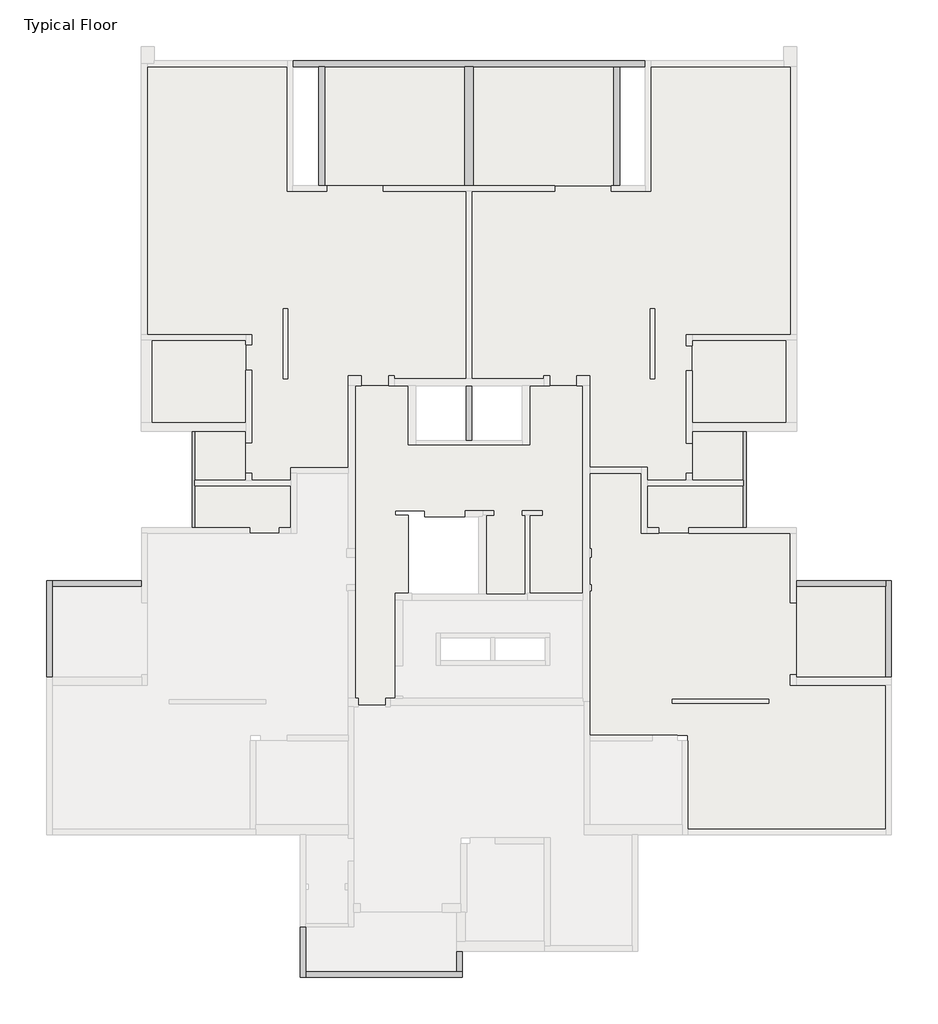
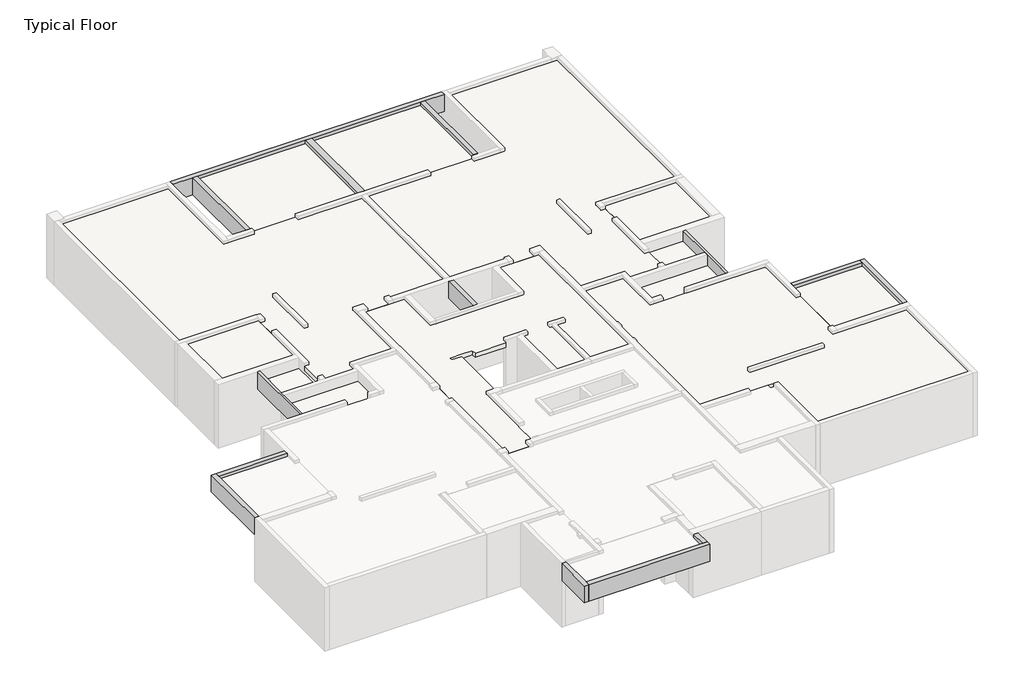
# One storey, part 4 of 4: 14 beams, 13 slabs.
"""IFC4 building model written with IfcOpenShell, lengths in millimetres."""

from ifc_helpers import new_model, si_unit, frame, origin, place, context, project, spatial, polyline, outline, extrude, faceted_brep, element, save

model = new_model("IFC4")

# Units and contexts
model_context = context("Model", 3, world=origin())
ifc_project = project(units=[si_unit("LENGTHUNIT", "METRE", prefix="MILLI")], contexts=[model_context])

# Site, building, storey
site = spatial("IfcSite", under=ifc_project)
building = spatial("IfcBuilding", under=site)
storey = spatial("IfcBuildingStorey", under=building, Name="Typical Floor", Elevation=3160.0)

# Beams
placement = place(None, origin())
element("IfcBeam", 1, ObjectType="Concrete Rectengular Beam : 10/80", at=placement, inside=storey, context=model_context, shape_type="Brep", body=[
    faceted_brep([(-4927.8090865, 3048.3506111, 3160.0), (-5027.8090865, 3048.3506111, 3160.0), (-5027.8090865, -271.5347538, 3160.0), (-4927.8090865, -271.5347538, 3160.0), (-4927.8090865, 1164.6693841, 3160.0), (-4927.8090865, 1364.6693841, 3160.0), (-4927.8090865, 3048.3506111, 2360.0), (-4927.8090865, 3048.3506111, 2510.0), (-4927.8090865, 3048.3506111, 2660.0), (-4927.8090865, -271.5347538, 2660.0), (-4927.8090865, -271.5347538, 2510.0), (-4927.8090865, -271.5347538, 2360.0), (-5027.8090865, 3048.3506111, 2360.0), (-5027.8090865, -271.5347538, 2360.0)], [[[0, 1, 2, 3, 4, 5]], [[6, 7, 8, 0, 5, 4, 3, 9, 10, 11]], [[12, 6, 11, 13]], [[1, 12, 13, 2]], [[1, 0, 8, 7, 6, 12]], [[3, 2, 13, 11, 10, 9]]]),
])
element("IfcBeam", 2, ObjectType="Concrete Rectengular Beam : 10/80", at=placement, inside=storey, context=model_context, shape_type="Brep", body=[
    faceted_brep([(14076.960118, 3048.3506111, 3160.0), (13976.960118, 3048.3506111, 3160.0), (13976.960118, 1364.6693841, 3160.0), (13976.960118, 1164.6693841, 3160.0), (13976.960118, -271.5348131, 3160.0), (14076.960118, -271.5348131, 3160.0), (14076.960118, 3048.3506111, 2360.0), (14076.960118, -271.5348131, 2360.0), (13976.960118, 3048.3506111, 2360.0), (13976.960118, -271.5348131, 2360.0), (13976.960118, 3048.3506111, 2660.0), (13976.960118, 3048.3506111, 2510.0), (13976.960118, -271.5348131, 2510.0), (13976.960118, -271.5348131, 2660.0)], [[[0, 1, 2, 3, 4, 5]], [[6, 0, 5, 7]], [[8, 6, 7, 9]], [[1, 10, 11, 8, 9, 12, 13, 4, 3, 2]], [[1, 0, 6, 8, 11, 10]], [[5, 4, 13, 12, 9, 7]]]),
])
element("IfcBeam", 3, ObjectType="Concrete Rectengular Beam : 20/80", at=placement, inside=storey, context=model_context, shape_type="Brep", body=[
    faceted_brep([(-9845.3223417, -2097.6508085, 3160.0), (-10045.3223417, -2097.6508085, 3160.0), (-10045.3223417, -5427.6243159, 3160.0), (-9845.3223417, -5427.6243159, 3160.0), (-9845.3223417, -2297.6508085, 3160.0), (-9845.3223417, -2097.6508085, 2360.0), (-9845.3223417, -5427.6243159, 3010.0), (-9845.3223417, -5427.6243159, 2810.0), (-9845.3223417, -5427.6243159, 2360.0), (-9845.3223417, -2297.6508085, 2360.0), (-10045.3223417, -2097.6508085, 2360.0), (-10045.3223417, -5427.6243159, 2360.0)], [[[0, 1, 2, 3, 4]], [[5, 0, 4, 3, 6, 7, 8, 9]], [[10, 5, 9, 8, 11]], [[1, 10, 11, 2]], [[1, 0, 5, 10]], [[3, 2, 11, 8, 7, 6]]]),
])
element("IfcBeam", 4, ObjectType="Concrete Rectengular Beam : 20/80", at=placement, inside=storey, context=model_context, shape_type="Brep", body=[
    faceted_brep([(-6765.3223417, -2097.6508085, 3160.0), (-6765.3223417, -2297.6508085, 3160.0), (-6765.3223417, -2297.6508085, 2360.0), (-6765.3223417, -2097.6508085, 2360.0), (-9845.3223417, -2097.6508085, 3160.0), (-9845.3223417, -2297.6508085, 3160.0), (-9845.3223417, -2297.6508085, 3010.0), (-9845.3223417, -2297.6508085, 2810.0), (-9845.3223417, -2297.6508085, 2360.0), (-9845.3223417, -2097.6508085, 2360.0)], [[[0, 1, 2, 3]], [[1, 0, 4, 5]], [[2, 1, 5, 6, 7, 8]], [[3, 2, 8, 9]], [[0, 3, 9, 4]], [[5, 4, 9, 8, 7, 6]]]),
])
element("IfcBeam", 5, ObjectType="Concrete Rectengular Beam : 20/80", at=placement, inside=storey, context=model_context, shape_type="Brep", body=[
    faceted_brep([(19089.4302812, -2097.6508085, 3160.0), (18889.4302812, -2097.6508085, 3160.0), (18889.4302812, -2297.6508085, 3160.0), (18889.4302812, -5431.5348131, 3160.0), (19089.4302812, -5431.5348131, 3160.0), (19089.4302812, -2097.6508085, 2360.0), (19089.4302812, -5431.5348131, 2360.0), (18889.4302812, -2097.6508085, 2360.0), (18889.4302812, -5431.5348131, 2360.0), (18889.4302812, -2297.6508085, 2360.0), (18889.4302812, -5431.5348131, 2810.0), (18889.4302812, -5431.5348131, 3010.0)], [[[0, 1, 2, 3, 4]], [[5, 0, 4, 6]], [[7, 5, 6, 8, 9]], [[1, 7, 9, 8, 10, 11, 3, 2]], [[1, 0, 5, 7]], [[4, 3, 11, 10, 8, 6]]]),
])
element("IfcBeam", 6, ObjectType="Concrete Rectengular Beam : 20/80", at=placement, inside=storey, context=model_context, shape_type="Brep", body=[
    faceted_brep([(15808.1220541, -2097.6508085, 3160.0), (15808.1220541, -2297.6508085, 3160.0), (18889.4302812, -2297.6508085, 3160.0), (18889.4302812, -2097.6508085, 3160.0), (15808.1220541, -2097.6508085, 2360.0), (18889.4302812, -2097.6508085, 2360.0), (15808.1220541, -2297.6508085, 2360.0), (18889.4302812, -2297.6508085, 2360.0), (15808.1220541, -2297.6508085, 3010.0), (15808.1220541, -2297.6508085, 2810.0), (18889.4302812, -2297.6508085, 2810.0), (18889.4302812, -2297.6508085, 3010.0)], [[[0, 1, 2, 3]], [[4, 0, 3, 5]], [[6, 4, 5, 7]], [[1, 8, 9, 6, 7, 10, 11, 2]], [[1, 0, 4, 6, 9, 8]], [[3, 2, 11, 10, 7, 5]]]),
])
element("IfcBeam", 7, ObjectType="Concrete Rectengular Beam : 20/80", at=placement, inside=storey, context=model_context, shape_type="Brep", body=[
    faceted_brep([(-1304.0660316, -15783.8829405, 3160.0), (-1104.0660316, -15783.8829405, 3160.0), (-1104.0660316, -15583.8829405, 3160.0), (-1104.0660316, -14027.6329213, 3160.0), (-1304.0660316, -14027.6329213, 3160.0), (-1304.0660316, -15783.8829405, 2360.0), (-1304.0660316, -14027.6329213, 2360.0), (-1104.0660316, -15783.8829405, 2360.0), (-1104.0660316, -14027.6329213, 2360.0), (-1104.0660316, -15583.8829405, 2360.0), (-1104.0660316, -14027.6329213, 2810.0), (-1104.0660316, -14027.6329213, 3010.0)], [[[0, 1, 2, 3, 4]], [[5, 0, 4, 6]], [[7, 5, 6, 8, 9]], [[1, 7, 9, 8, 10, 11, 3, 2]], [[4, 3, 11, 10, 8, 6]], [[1, 0, 5, 7]]]),
])
element("IfcBeam", 8, ObjectType="Concrete Rectengular Beam : 20/80", at=placement, inside=storey, context=model_context, shape_type="Brep", body=[
    faceted_brep([(4293.8641143, -15783.8829405, 3160.0), (4293.8641143, -15583.8829405, 3160.0), (4093.8641143, -15583.8829405, 3160.0), (-1104.0660316, -15583.8829405, 3160.0), (-1104.0660316, -15783.8829405, 3160.0), (4293.8641143, -15783.8829405, 2360.0), (-1104.0660316, -15783.8829405, 2360.0), (4293.8641143, -15583.8829405, 2360.0), (-1104.0660316, -15583.8829405, 2360.0), (4093.8641143, -15583.8829405, 2360.0), (-1104.0660316, -15583.8829405, 2810.0), (-1104.0660316, -15583.8829405, 3010.0)], [[[0, 1, 2, 3, 4]], [[5, 0, 4, 6]], [[7, 5, 6, 8, 9]], [[1, 7, 9, 8, 10, 11, 3, 2]], [[1, 0, 5, 7]], [[4, 3, 11, 10, 8, 6]]]),
])
element("IfcBeam", 9, ObjectType="Concrete Rectengular Beam : 20/80", at=placement, inside=storey, context=model_context, shape_type="Brep", body=[
    faceted_brep([(4293.8641143, -14884.0137597, 3160.0), (4093.8641143, -14884.0137597, 3160.0), (4093.8641143, -15583.8829405, 3160.0), (4293.8641143, -15583.8829405, 3160.0), (4293.8641143, -14884.0137597, 2360.0), (4293.8641143, -15583.8829405, 2360.0), (4093.8641143, -14884.0137597, 2360.0), (4093.8641143, -15583.8829405, 2360.0), (4093.8641143, -15583.8829405, 2810.0), (4093.8641143, -15583.8829405, 3010.0)], [[[0, 1, 2, 3]], [[4, 0, 3, 5]], [[6, 4, 5, 7]], [[1, 6, 7, 8, 9, 2]], [[1, 0, 4, 6]], [[3, 2, 9, 8, 7, 5]]]),
])
element("IfcBeam", 10, ObjectType="Concrete Rectengular Beam : 20/80", at=placement, inside=storey, context=model_context, shape_type="Brep", body=[
    faceted_brep([(-1550.9499448, 15824.626844, 3160.0), (-1550.9499448, 15624.626844, 3160.0), (-650.9499448, 15624.626844, 3160.0), (-450.9499448, 15624.626844, 3160.0), (4369.0500552, 15624.626844, 3160.0), (4669.0500552, 15624.626844, 3160.0), (9515.057825, 15624.626844, 3160.0), (9715.057825, 15624.626844, 3160.0), (10595.057825, 15624.626844, 3160.0), (10595.057825, 15824.626844, 3160.0), (-1550.9499448, 15624.626844, 2360.0), (-650.9499448, 15624.626844, 2360.0), (-450.9499448, 15624.626844, 2360.0), (4369.0500552, 15624.626844, 2360.0), (4669.0500552, 15624.626844, 2360.0), (9515.057825, 15624.626844, 2360.0), (9715.057825, 15624.626844, 2360.0), (10595.057825, 15624.626844, 2360.0), (-1550.9499448, 15824.626844, 2360.0), (10595.057825, 15824.626844, 2360.0)], [[[0, 1, 2, 3, 4, 5, 6, 7, 8, 9]], [[1, 10, 11, 12, 13, 14, 15, 16, 17, 8, 7, 6, 5, 4, 3, 2]], [[10, 18, 19, 17, 16, 15, 14, 13, 12, 11]], [[18, 0, 9, 19]], [[1, 0, 18, 10]], [[9, 8, 17, 19]]]),
])
element("IfcBeam", 11, ObjectType="Concrete Rectengular Beam : 20/80", at=placement, inside=storey, context=model_context, shape_type="Brep", body=[
    faceted_brep([(-650.9499448, 11524.9195447, 3160.0), (-450.9499448, 11524.9195447, 3160.0), (-450.9499448, 15624.626844, 3160.0), (-650.9499448, 15624.626844, 3160.0), (-650.9499448, 11524.9195447, 2360.0), (-650.9499448, 15624.626844, 2360.0), (-450.9499448, 11524.9195447, 2360.0), (-450.9499448, 15624.626844, 2360.0), (-450.9499448, 11524.9195447, 3010.0), (-450.9499448, 11524.9195447, 2810.0), (-450.9499448, 15624.626844, 2810.0), (-450.9499448, 15624.626844, 3010.0)], [[[0, 1, 2, 3]], [[4, 0, 3, 5]], [[6, 4, 5, 7]], [[1, 8, 9, 6, 7, 10, 11, 2]], [[1, 0, 4, 6, 9, 8]], [[3, 2, 11, 10, 7, 5]]]),
])
element("IfcBeam", 12, ObjectType="Concrete Rectengular Beam : 20/80", at=placement, inside=storey, context=model_context, shape_type="Brep", body=[
    faceted_brep([(9515.057825, 11524.9195447, 3160.0), (9715.057825, 11524.9195447, 3160.0), (9715.057825, 15624.626844, 3160.0), (9515.057825, 15624.626844, 3160.0), (9515.057825, 11524.9195447, 2360.0), (9515.057825, 11524.9195447, 2810.0), (9515.057825, 11524.9195447, 3010.0), (9515.057825, 15624.626844, 3010.0), (9515.057825, 15624.626844, 2810.0), (9515.057825, 15624.626844, 2360.0), (9715.057825, 11524.9195447, 2360.0), (9715.057825, 15624.626844, 2360.0)], [[[0, 1, 2, 3]], [[4, 5, 6, 0, 3, 7, 8, 9]], [[10, 4, 9, 11]], [[1, 10, 11, 2]], [[1, 0, 6, 5, 4, 10]], [[3, 2, 11, 9, 8, 7]]]),
])
element("IfcBeam", 13, ObjectType="Concrete Rectengular Beam : 20/80", at=placement, inside=storey, context=model_context, shape_type="SweptSolid", body=[
    extrude(outline(polyline([(4422.0544149, 4615.5631538), (4622.0544149, 4615.5631538), (4622.0544149, 2732.4743311), (4422.0544149, 2732.4743311), (4422.0544149, 4615.5631538)])), frame((0.0, 0.0, 2360.0), z_axis=(0.0, 0.0, 1.0), x_axis=(1.0, 0.0, 0.0)), (0.0, 0.0, 1.0), 800.0),
])
element("IfcBeam", 14, ObjectType="Concrete Rectengular Beam : 30/80", at=placement, inside=storey, context=model_context, shape_type="Brep", body=[
    faceted_brep([(4369.0500552, 11524.9195447, 3160.0), (4669.0500552, 11524.9195447, 3160.0), (4669.0500552, 15624.626844, 3160.0), (4369.0500552, 15624.626844, 3160.0), (4369.0500552, 11524.9195447, 2360.0), (4369.0500552, 11524.9195447, 2810.0), (4369.0500552, 11524.9195447, 3010.0), (4369.0500552, 15624.626844, 3010.0), (4369.0500552, 15624.626844, 2810.0), (4369.0500552, 15624.626844, 2360.0), (4669.0500552, 11524.9195447, 2360.0), (4669.0500552, 15624.626844, 2360.0), (4669.0500552, 11524.9195447, 3010.0), (4669.0500552, 11524.9195447, 2810.0), (4669.0500552, 15624.626844, 2810.0), (4669.0500552, 15624.626844, 3010.0)], [[[0, 1, 2, 3]], [[4, 5, 6, 0, 3, 7, 8, 9]], [[10, 4, 9, 11]], [[1, 12, 13, 10, 11, 14, 15, 2]], [[1, 0, 6, 5, 4, 10, 13, 12]], [[3, 2, 15, 14, 11, 9, 8, 7]]]),
])

# Slabs
element("IfcSlab", 15, ObjectType="D=20", at=placement, inside=storey, context=model_context, shape_type="Brep", body=[
    faceted_brep([(18889.4302812, -10669.1739201, 2810.0), (12069.8374389, -10669.1739201, 2810.0), (12069.8374389, -7625.251138, 2810.0), (12069.8374389, -7425.251138, 2810.0), (11709.8374389, -7425.251138, 2810.0), (10849.2361919, -7425.251138, 2810.0), (8689.2361919, -7425.251138, 2810.0), (8689.2361919, -2440.6761415, 2810.0), (8740.4562765, -2440.6761415, 2810.0), (8740.4562765, -2240.6761415, 2810.0), (8689.2361919, -2240.6761415, 2810.0), (8689.2361919, -1298.8355577, 2810.0), (8740.4562765, -1298.8355577, 2810.0), (8740.4562765, -998.8355577, 2810.0), (8689.2361919, -998.8355577, 2810.0), (8689.2361919, 1602.6523966, 2810.0), (8692.9791875, 1602.6523966, 2810.0), (10462.1205752, 1602.6523966, 2810.0), (10462.1205752, -471.5348131, 2810.0), (10662.1205752, -471.5348131, 2810.0), (11062.1205752, -471.5348131, 2810.0), (12108.1220541, -471.5348131, 2810.0), (15608.1220541, -471.5348131, 2810.0), (15608.1220541, -2868.5711301, 2810.0), (15808.1220541, -2868.5711301, 2810.0), (15808.1220541, -5351.6580536, 2810.0), (15608.1220541, -5351.6580536, 2810.0), (15608.1220541, -5711.5348131, 2810.0), (15808.1220541, -5711.5348131, 2810.0), (18889.4302812, -5711.5348131, 2810.0), (11536.8984681, -6331.4817686, 2810.0), (14866.281411, -6331.4817686, 2810.0), (14866.281411, -6181.4817686, 2810.0), (11536.8984681, -6181.4817686, 2810.0), (12069.8374389, -10669.1739201, 3010.0), (18889.4302812, -10669.1739201, 3010.0), (18889.4302812, -5711.5348131, 3010.0), (15808.1220541, -5711.5348131, 3010.0), (15608.1220541, -5711.5348131, 3010.0), (15608.1220541, -5351.6580536, 3010.0), (15808.1220541, -5351.6580536, 3010.0), (15808.1220541, -2868.5711301, 3010.0), (15608.1220541, -2868.5711301, 3010.0), (15608.1220541, -471.5348131, 3010.0), (12108.1220541, -471.5348131, 3010.0), (11062.1205752, -471.5348131, 3010.0), (10662.1205752, -471.5348131, 3010.0), (10462.1205752, -471.5348131, 3010.0), (10462.1205752, 1602.6523966, 3010.0), (8692.9791875, 1602.6523966, 3010.0), (8689.2361919, 1602.6523966, 3010.0), (8689.2361919, -998.8355577, 3010.0), (8740.4562765, -998.8355577, 3010.0), (8740.4562765, -1298.8355577, 3010.0), (8689.2361919, -1298.8355577, 3010.0), (8689.2361919, -2240.6761415, 3010.0), (8740.4562765, -2240.6761415, 3010.0), (8740.4562765, -2440.6761415, 3010.0), (8689.2361919, -2440.6761415, 3010.0), (8689.2361919, -7425.251138, 3010.0), (10849.2361919, -7425.251138, 3010.0), (11709.8374389, -7425.251138, 3010.0), (12069.8374389, -7425.251138, 3010.0), (12069.8374389, -7625.251138, 3010.0), (14866.281411, -6331.4817686, 3010.0), (11536.8984681, -6331.4817686, 3010.0), (11536.8984681, -6181.4817686, 3010.0), (14866.281411, -6181.4817686, 3010.0)], [[[0, 1, 2, 3, 4, 5, 6, 7, 8, 9, 10, 11, 12, 13, 14, 15, 16, 17, 18, 19, 20, 21, 22, 23, 24, 25, 26, 27, 28, 29], [30, 31, 32, 33]], [[34, 35, 36, 37, 38, 39, 40, 41, 42, 43, 44, 45, 46, 47, 48, 49, 50, 51, 52, 53, 54, 55, 56, 57, 58, 59, 60, 61, 62, 63], [64, 65, 66, 67]], [[1, 0, 35, 34]], [[1, 34, 63, 62, 3, 2]], [[3, 62, 61, 60, 59, 6, 5, 4]], [[7, 6, 59, 58]], [[8, 7, 58, 57]], [[9, 8, 57, 56]], [[10, 9, 56, 55]], [[11, 10, 55, 54]], [[12, 11, 54, 53]], [[13, 12, 53, 52]], [[14, 13, 52, 51]], [[15, 14, 51, 50]], [[16, 15, 50, 49]], [[17, 16, 49, 48]], [[18, 17, 48, 47]], [[18, 47, 46, 45, 44, 43, 22, 21, 20, 19]], [[23, 22, 43, 42]], [[24, 23, 42, 41]], [[25, 24, 41, 40]], [[26, 25, 40, 39]], [[27, 26, 39, 38]], [[27, 38, 37, 36, 29, 28]], [[0, 29, 36, 35]], [[31, 30, 65, 64]], [[33, 32, 67, 66]], [[32, 31, 64, 67]], [[30, 33, 66, 65]]]),
])
element("IfcSlab", 16, ObjectType="D=20", at=placement, inside=storey, context=model_context, shape_type="Brep", body=[
    faceted_brep([(6609.8903055, 2582.4743311, 2810.0), (6609.8903055, 4615.5631538, 2810.0), (7104.8461452, 4615.5631538, 2810.0), (7304.8461452, 4615.5631538, 2810.0), (8239.2361919, 4615.5631538, 2810.0), (8239.2361919, 4613.0861241, 2810.0), (8439.2361919, 4613.0861241, 2810.0), (8439.2361919, -2526.1363023, 2810.0), (6609.8903055, -2526.1363023, 2810.0), (6609.8903055, 156.3601755, 2810.0), (7056.7750495, 156.3601755, 2810.0), (7056.7750495, 306.3601755, 2810.0), (6362.4114361, 306.3601755, 2810.0), (6362.4114361, 156.3601755, 2810.0), (6459.8903055, 156.3601755, 2810.0), (6459.8903055, -2576.1363023, 2810.0), (5116.7132216, -2576.1363023, 2810.0), (5116.7132216, 156.3601755, 2810.0), (5376.7132216, 156.3601755, 2810.0), (5376.7132216, 306.3601755, 2810.0), (4991.7132216, 306.3601755, 2810.0), (4391.7132216, 306.3601755, 2810.0), (4391.7132216, 106.3601755, 2810.0), (2996.6955539, 106.3601755, 2810.0), (2996.6955539, 306.3601755, 2810.0), (2556.6955539, 306.3601755, 2810.0), (1986.6955539, 306.3601755, 2810.0), (1986.6955539, 156.3601755, 2810.0), (2431.6955539, 156.3601755, 2810.0), (2431.6955539, -2526.1363023, 2810.0), (1987.3338395, -2526.1363023, 2810.0), (1987.3338395, -2776.1363023, 2810.0), (1987.3338395, -5031.1363023, 2810.0), (1987.3338395, -6084.0047389, 2810.0), (1987.3338395, -6150.4733638, 2810.0), (1804.8990117, -6150.4733638, 2810.0), (1644.8990117, -6150.4733638, 2810.0), (1644.8990117, -6400.4733638, 2810.0), (703.0584279, -6400.4733638, 2810.0), (703.0584279, -6150.4733638, 2810.0), (603.6524939, -6150.4733638, 2810.0), (603.6524939, -2240.6761415, 2810.0), (603.0274939, -2240.6761415, 2810.0), (603.0274939, -1298.8355577, 2810.0), (603.0274939, 4618.0861241, 2810.0), (803.0602083, 4618.0861241, 2810.0), (1749.3507084, 4618.0861241, 2810.0), (1749.3507084, 4615.5631538, 2810.0), (2434.2185243, 4615.5631538, 2810.0), (2434.2185243, 2582.4743311, 2810.0), (2684.2185243, 2582.4743311, 2810.0), (6359.8903055, 2582.4743311, 2810.0), (6609.8903055, 4615.5631538, 3010.0), (6609.8903055, 2582.4743311, 3010.0), (6359.8903055, 2582.4743311, 3010.0), (2684.2185243, 2582.4743311, 3010.0), (2434.2185243, 2582.4743311, 3010.0), (2434.2185243, 4615.5631538, 3010.0), (1749.3507084, 4615.5631538, 3010.0), (1749.3507084, 4618.0861241, 3010.0), (803.0602083, 4618.0861241, 3010.0), (603.0274939, 4618.0861241, 3010.0), (603.0274939, -1298.8355577, 3010.0), (603.0274939, -2240.6761415, 3010.0), (603.6524939, -2240.6761415, 3010.0), (603.6524939, -6150.4733638, 3010.0), (703.0584279, -6150.4733638, 3010.0), (703.0584279, -6400.4733638, 3010.0), (1644.8990117, -6400.4733638, 3010.0), (1644.8990117, -6150.4733638, 3010.0), (1804.8990117, -6150.4733638, 3010.0), (1987.3338395, -6150.4733638, 3010.0), (1987.3338395, -6084.0047389, 3010.0), (1987.3338395, -5031.1363023, 3010.0), (1987.3338395, -2776.1363023, 3010.0), (1987.3338395, -2526.1363023, 3010.0), (2431.6955539, -2526.1363023, 3010.0), (2431.6955539, 156.3601755, 3010.0), (1986.6955539, 156.3601755, 3010.0), (1986.6955539, 306.3601755, 3010.0), (2556.6955539, 306.3601755, 3010.0), (2996.6955539, 306.3601755, 3010.0), (2996.6955539, 106.3601755, 3010.0), (4391.7132216, 106.3601755, 3010.0), (4391.7132216, 306.3601755, 3010.0), (4991.7132216, 306.3601755, 3010.0), (5376.7132216, 306.3601755, 3010.0), (5376.7132216, 156.3601755, 3010.0), (5116.7132216, 156.3601755, 3010.0), (5116.7132216, -2576.1363023, 3010.0), (6459.8903055, -2576.1363023, 3010.0), (6459.8903055, 156.3601755, 3010.0), (6362.4114361, 156.3601755, 3010.0), (6362.4114361, 306.3601755, 3010.0), (7056.7750495, 306.3601755, 3010.0), (7056.7750495, 156.3601755, 3010.0), (6609.8903055, 156.3601755, 3010.0), (6609.8903055, -2526.1363023, 3010.0), (8439.2361919, -2526.1363023, 3010.0), (8439.2361919, 4613.0861241, 3010.0), (8239.2361919, 4613.0861241, 3010.0), (8239.2361919, 4615.5631538, 3010.0), (7304.8461452, 4615.5631538, 3010.0), (7104.8461452, 4615.5631538, 3010.0)], [[[0, 1, 2, 3, 4, 5, 6, 7, 8, 9, 10, 11, 12, 13, 14, 15, 16, 17, 18, 19, 20, 21, 22, 23, 24, 25, 26, 27, 28, 29, 30, 31, 32, 33, 34, 35, 36, 37, 38, 39, 40, 41, 42, 43, 44, 45, 46, 47, 48, 49, 50, 51]], [[52, 53, 54, 55, 56, 57, 58, 59, 60, 61, 62, 63, 64, 65, 66, 67, 68, 69, 70, 71, 72, 73, 74, 75, 76, 77, 78, 79, 80, 81, 82, 83, 84, 85, 86, 87, 88, 89, 90, 91, 92, 93, 94, 95, 96, 97, 98, 99, 100, 101, 102, 103]], [[39, 66, 65, 40]], [[61, 44, 43, 42, 63, 62]], [[44, 61, 60, 59, 46, 45]], [[56, 49, 48, 57]], [[49, 56, 55, 54, 53, 0, 51, 50]], [[1, 0, 53, 52]], [[1, 52, 103, 102, 101, 4, 3, 2]], [[98, 7, 6, 99]], [[8, 7, 98, 97]], [[9, 8, 97, 96]], [[10, 9, 96, 95]], [[11, 10, 95, 94]], [[27, 26, 79, 78]], [[28, 27, 78, 77]], [[29, 28, 77, 76]], [[30, 29, 76, 75]], [[30, 75, 74, 73, 72, 33, 32, 31]], [[34, 33, 72, 71]], [[34, 71, 70, 69, 36, 35]], [[37, 36, 69, 68]], [[38, 37, 68, 67]], [[39, 38, 67, 66]], [[57, 48, 47, 58]], [[47, 46, 59, 58]], [[5, 4, 101, 100]], [[6, 5, 100, 99]], [[40, 65, 64, 41]], [[84, 21, 20, 19, 86, 85]], [[22, 21, 84, 83]], [[23, 22, 83, 82]], [[24, 23, 82, 81]], [[24, 81, 80, 79, 26, 25]], [[41, 64, 63, 42]], [[12, 11, 94, 93]], [[13, 12, 93, 92]], [[14, 13, 92, 91]], [[15, 14, 91, 90]], [[16, 15, 90, 89]], [[17, 16, 89, 88]], [[18, 17, 88, 87]], [[19, 18, 87, 86]]]),
])
element("IfcSlab", 17, ObjectType="D=20", at=placement, inside=storey, context=model_context, shape_type="Brep", body=[
    faceted_brep([(-3168.7557226, 6187.8215778, 2810.0), (-3168.7557226, 6027.8215778, 2810.0), (-3168.7557226, 5158.3506111, 2810.0), (-3168.7557226, 3348.3506111, 2810.0), (-6424.1013669, 3348.3506111, 2810.0), (-6424.1013669, 6187.8215778, 2810.0), (-3168.7557226, 6187.8215778, 3010.0), (-6424.1013669, 6187.8215778, 3010.0), (-6424.1013669, 3348.3506111, 3010.0), (-3168.7557226, 3348.3506111, 3010.0), (-3168.7557226, 5158.3506111, 3010.0), (-3168.7557226, 6027.8215778, 3010.0)], [[[0, 1, 2, 3, 4, 5]], [[6, 7, 8, 9, 10, 11]], [[3, 2, 1, 0, 6, 11, 10, 9]], [[4, 3, 9, 8]], [[5, 4, 8, 7]], [[0, 5, 7, 6]]]),
])
element("IfcSlab", 18, ObjectType="D=20", at=placement, inside=storey, context=model_context, shape_type="SweptSolid", body=[
    extrude(outline(polyline([(12222.3603499, 5144.6693841), (12221.7662246, 5144.6693841), (12221.7662246, 6007.8215778), (12222.3603499, 6007.8215778), (12222.3603499, 6187.8198567), (15467.6160713, 6187.8198567), (15467.6160713, 3348.3506111), (12222.3603499, 3348.3506111), (12222.3603499, 5144.6693841)])), frame((0.0, 0.0, 2810.0), z_axis=(0.0, 0.0, 1.0), x_axis=(1.0, 0.0, 0.0)), (0.0, 0.0, 1.0), 200.0),
])
element("IfcSlab", 19, ObjectType="D=20", at=placement, inside=storey, context=model_context, shape_type="Brep", body=[
    faceted_brep([(-3168.7557226, 1604.6693841, 2810.0), (-3168.7557226, 2648.3506111, 2810.0), (-2968.7557226, 2648.3506111, 2810.0), (-2968.7557226, 5158.3506111, 2810.0), (-3168.7557226, 5158.3506111, 2810.0), (-3168.7557226, 6027.8215778, 2810.0), (-2968.7557226, 6027.8215778, 2810.0), (-2968.7557226, 6387.8215778, 2810.0), (-3168.7557226, 6387.8215778, 2810.0), (-6574.1013669, 6387.8215778, 2810.0), (-6574.1013669, 15624.626844, 2810.0), (-1750.9499448, 15624.626844, 2810.0), (-1750.9499448, 11324.9195447, 2810.0), (-1550.9499448, 11324.9195447, 2810.0), (-390.7110009, 11324.9195447, 2810.0), (-390.7110009, 11524.9195447, 2810.0), (1568.9345892, 11524.9195447, 2810.0), (1568.9345892, 11324.9195447, 2810.0), (4422.3514479, 11324.9195447, 2810.0), (4422.3514479, 4865.5631538, 2810.0), (1949.3507084, 4865.5631538, 2810.0), (1949.3507084, 4970.0149098, 2810.0), (1749.3507084, 4970.0149098, 2810.0), (1749.3507084, 4618.0861241, 2810.0), (803.0602083, 4618.0861241, 2810.0), (803.0602083, 4970.0149098, 2810.0), (353.0602083, 4970.0149098, 2810.0), (353.0602083, 4618.0861241, 2810.0), (353.0602083, 1802.0583306, 2810.0), (-1618.0126357, 1802.0583306, 2810.0), (-1618.0126357, 1602.0583306, 2810.0), (-1618.0126357, 1364.6693841, 2810.0), (-2968.7557226, 1364.6693841, 2810.0), (-2968.7557226, 1604.6693841, 2810.0), (-1883.8880254, 7281.591066, 2810.0), (-1883.8880254, 4865.5631538, 2810.0), (-1733.8880254, 4865.5631538, 2810.0), (-1733.8880254, 7281.591066, 2810.0), (-3168.7557226, 2648.3506111, 3010.0), (-3168.7557226, 1604.6693841, 3010.0), (-2968.7557226, 1604.6693841, 3010.0), (-2968.7557226, 1364.6693841, 3010.0), (-1618.0126357, 1364.6693841, 3010.0), (-1618.0126357, 1602.0583306, 3010.0), (-1618.0126357, 1802.0583306, 3010.0), (353.0602083, 1802.0583306, 3010.0), (353.0602083, 4618.0861241, 3010.0), (353.0602083, 4970.0149098, 3010.0), (803.0602083, 4970.0149098, 3010.0), (803.0602083, 4618.0861241, 3010.0), (1749.3507084, 4618.0861241, 3010.0), (1749.3507084, 4970.0149098, 3010.0), (1949.3507084, 4970.0149098, 3010.0), (1949.3507084, 4865.5631538, 3010.0), (4422.3514479, 4865.5631538, 3010.0), (4422.3514479, 11324.9195447, 3010.0), (1568.9345892, 11324.9195447, 3010.0), (1568.9345892, 11524.9195447, 3010.0), (-390.7110009, 11524.9195447, 3010.0), (-390.7110009, 11324.9195447, 3010.0), (-1550.9499448, 11324.9195447, 3010.0), (-1750.9499448, 11324.9195447, 3010.0), (-1750.9499448, 15624.626844, 3010.0), (-6574.1013669, 15624.626844, 3010.0), (-6574.1013669, 6387.8215778, 3010.0), (-3168.7557226, 6387.8215778, 3010.0), (-2968.7557226, 6387.8215778, 3010.0), (-2968.7557226, 6027.8215778, 3010.0), (-3168.7557226, 6027.8215778, 3010.0), (-3168.7557226, 5158.3506111, 3010.0), (-2968.7557226, 5158.3506111, 3010.0), (-2968.7557226, 2648.3506111, 3010.0), (-1883.8880254, 4865.5631538, 3010.0), (-1883.8880254, 7281.591066, 3010.0), (-1733.8880254, 7281.591066, 3010.0), (-1733.8880254, 4865.5631538, 3010.0)], [[[0, 1, 2, 3, 4, 5, 6, 7, 8, 9, 10, 11, 12, 13, 14, 15, 16, 17, 18, 19, 20, 21, 22, 23, 24, 25, 26, 27, 28, 29, 30, 31, 32, 33], [34, 35, 36, 37]], [[38, 39, 40, 41, 42, 43, 44, 45, 46, 47, 48, 49, 50, 51, 52, 53, 54, 55, 56, 57, 58, 59, 60, 61, 62, 63, 64, 65, 66, 67, 68, 69, 70, 71], [72, 73, 74, 75]], [[1, 0, 39, 38]], [[2, 1, 38, 71]], [[3, 2, 71, 70]], [[4, 3, 70, 69]], [[5, 4, 69, 68]], [[6, 5, 68, 67]], [[7, 6, 67, 66]], [[7, 66, 65, 64, 9, 8]], [[10, 9, 64, 63]], [[11, 10, 63, 62]], [[12, 11, 62, 61]], [[12, 61, 60, 59, 14, 13]], [[15, 14, 59, 58]], [[16, 15, 58, 57]], [[17, 16, 57, 56]], [[18, 17, 56, 55]], [[19, 18, 55, 54]], [[20, 19, 54, 53]], [[21, 20, 53, 52]], [[22, 21, 52, 51]], [[23, 22, 51, 50]], [[24, 23, 50, 49]], [[25, 24, 49, 48]], [[26, 25, 48, 47]], [[26, 47, 46, 45, 28, 27]], [[29, 28, 45, 44]], [[29, 44, 43, 42, 31, 30]], [[32, 31, 42, 41]], [[33, 32, 41, 40]], [[0, 33, 40, 39]], [[35, 34, 73, 72]], [[37, 36, 75, 74]], [[36, 35, 72, 75]], [[34, 37, 74, 73]]]),
])
element("IfcSlab", 20, ObjectType="D=20", at=placement, inside=storey, context=model_context, shape_type="Brep", body=[
    faceted_brep([(4622.3514479, 11324.9195447, 2810.0), (7485.2622644, 11324.9195447, 2810.0), (7485.2622644, 11524.9195447, 2810.0), (9434.8198306, 11524.9195447, 2810.0), (9434.8198306, 11324.9195447, 2810.0), (10595.057825, 11324.9195447, 2810.0), (10795.057825, 11324.9195447, 2810.0), (10795.057825, 15624.6267847, 2810.0), (15617.6160713, 15624.6267847, 2810.0), (15617.6160713, 6387.8215778, 2810.0), (12222.3603499, 6387.8215778, 2810.0), (12022.3603499, 6387.8215778, 2810.0), (12022.3603499, 6007.8215778, 2810.0), (12221.7662246, 6007.8215778, 2810.0), (12221.7662246, 5144.6693841, 2810.0), (12022.3603499, 5144.6693841, 2810.0), (12022.3603499, 2644.6693841, 2810.0), (12222.3603499, 2644.6693841, 2810.0), (12222.3603499, 1602.6523966, 2810.0), (12022.3603499, 1602.6523966, 2810.0), (12022.3603499, 1364.6693841, 2810.0), (10662.1205752, 1364.6693841, 2810.0), (10662.1205752, 1802.6523966, 2810.0), (10462.1205752, 1802.6523966, 2810.0), (8689.2361919, 1802.6523966, 2810.0), (8689.2361919, 4613.0861241, 2810.0), (8689.2361919, 4965.0149098, 2810.0), (8239.2361919, 4965.0149098, 2810.0), (8239.2361919, 4615.5631538, 2810.0), (7304.8461452, 4615.5631538, 2810.0), (7304.8461452, 4970.0149098, 2810.0), (7104.8461452, 4970.0149098, 2810.0), (7104.8461452, 4865.5631538, 2810.0), (4622.3514479, 4865.5631538, 2810.0), (10776.0680695, 7281.591066, 2810.0), (10776.0680695, 4865.5631538, 2810.0), (10926.0680695, 4865.5631538, 2810.0), (10926.0680695, 7281.591066, 2810.0), (7485.2622644, 11324.9195447, 3010.0), (4622.3514479, 11324.9195447, 3010.0), (4622.3514479, 4865.5631538, 3010.0), (7104.8461452, 4865.5631538, 3010.0), (7104.8461452, 4970.0149098, 3010.0), (7304.8461452, 4970.0149098, 3010.0), (7304.8461452, 4615.5631538, 3010.0), (8239.2361919, 4615.5631538, 3010.0), (8239.2361919, 4965.0149098, 3010.0), (8689.2361919, 4965.0149098, 3010.0), (8689.2361919, 4613.0861241, 3010.0), (8689.2361919, 1802.6523966, 3010.0), (10462.1205752, 1802.6523966, 3010.0), (10662.1205752, 1802.6523966, 3010.0), (10662.1205752, 1364.6693841, 3010.0), (12022.3603499, 1364.6693841, 3010.0), (12022.3603499, 1602.6523966, 3010.0), (12222.3603499, 1602.6523966, 3010.0), (12222.3603499, 2644.6693841, 3010.0), (12022.3603499, 2644.6693841, 3010.0), (12022.3603499, 5144.6693841, 3010.0), (12221.7662246, 5144.6693841, 3010.0), (12221.7662246, 6007.8215778, 3010.0), (12022.3603499, 6007.8215778, 3010.0), (12022.3603499, 6387.8215778, 3010.0), (12222.3603499, 6387.8215778, 3010.0), (15617.6160713, 6387.8215778, 3010.0), (15617.6160713, 15624.6267847, 3010.0), (10795.057825, 15624.6267847, 3010.0), (10795.057825, 11324.9195447, 3010.0), (10595.057825, 11324.9195447, 3010.0), (9434.8198306, 11324.9195447, 3010.0), (9434.8198306, 11524.9195447, 3010.0), (7485.2622644, 11524.9195447, 3010.0), (10776.0680695, 4865.5631538, 3010.0), (10776.0680695, 7281.591066, 3010.0), (10926.0680695, 7281.591066, 3010.0), (10926.0680695, 4865.5631538, 3010.0)], [[[0, 1, 2, 3, 4, 5, 6, 7, 8, 9, 10, 11, 12, 13, 14, 15, 16, 17, 18, 19, 20, 21, 22, 23, 24, 25, 26, 27, 28, 29, 30, 31, 32, 33], [34, 35, 36, 37]], [[38, 39, 40, 41, 42, 43, 44, 45, 46, 47, 48, 49, 50, 51, 52, 53, 54, 55, 56, 57, 58, 59, 60, 61, 62, 63, 64, 65, 66, 67, 68, 69, 70, 71], [72, 73, 74, 75]], [[1, 0, 39, 38]], [[2, 1, 38, 71]], [[3, 2, 71, 70]], [[4, 3, 70, 69]], [[4, 69, 68, 67, 6, 5]], [[7, 6, 67, 66]], [[8, 7, 66, 65]], [[9, 8, 65, 64]], [[9, 64, 63, 62, 11, 10]], [[12, 11, 62, 61]], [[13, 12, 61, 60]], [[14, 13, 60, 59]], [[15, 14, 59, 58]], [[16, 15, 58, 57]], [[17, 16, 57, 56]], [[18, 17, 56, 55]], [[19, 18, 55, 54]], [[20, 19, 54, 53]], [[21, 20, 53, 52]], [[22, 21, 52, 51]], [[22, 51, 50, 49, 24, 23]], [[24, 49, 48, 47, 26, 25]], [[27, 26, 47, 46]], [[28, 27, 46, 45]], [[29, 28, 45, 44]], [[30, 29, 44, 43]], [[31, 30, 43, 42]], [[32, 31, 42, 41]], [[33, 32, 41, 40]], [[0, 33, 40, 39]], [[35, 34, 73, 72]], [[37, 36, 75, 74]], [[36, 35, 72, 75]], [[34, 37, 74, 73]]]),
])
element("IfcSlab", 21, ObjectType="D=20", at=placement, inside=storey, context=model_context, shape_type="Brep", body=[
    faceted_brep([(4369.0500552, 15624.626844, 2810.0), (4369.0500552, 11524.9195447, 2810.0), (1568.9345892, 11524.9195447, 2810.0), (-390.7110009, 11524.9195447, 2810.0), (-450.9499448, 11524.9195447, 2810.0), (-450.9499448, 15624.626844, 2810.0), (4369.0500552, 11524.9195447, 3010.0), (4369.0500552, 15624.626844, 3010.0), (-450.9499448, 15624.626844, 3010.0), (-450.9499448, 11524.9195447, 3010.0), (-390.7110009, 11524.9195447, 3010.0), (1568.9345892, 11524.9195447, 3010.0)], [[[0, 1, 2, 3, 4, 5]], [[6, 7, 8, 9, 10, 11]], [[1, 0, 7, 6]], [[1, 6, 11, 10, 9, 4, 3, 2]], [[5, 4, 9, 8]], [[0, 5, 8, 7]]]),
])
element("IfcSlab", 22, ObjectType="D=20", at=placement, inside=storey, context=model_context, shape_type="Brep", body=[
    faceted_brep([(9515.057825, 15624.626844, 2810.0), (9515.057825, 11524.9195447, 2810.0), (9434.8198306, 11524.9195447, 2810.0), (7485.2622644, 11524.9195447, 2810.0), (4669.0500552, 11524.9195447, 2810.0), (4669.0500552, 15624.626844, 2810.0), (9515.057825, 11524.9195447, 3010.0), (9515.057825, 15624.626844, 3010.0), (4669.0500552, 15624.626844, 3010.0), (4669.0500552, 11524.9195447, 3010.0), (7485.2622644, 11524.9195447, 3010.0), (9434.8198306, 11524.9195447, 3010.0)], [[[0, 1, 2, 3, 4, 5]], [[6, 7, 8, 9, 10, 11]], [[1, 0, 7, 6]], [[1, 6, 11, 10, 9, 4, 3, 2]], [[5, 4, 9, 8]], [[0, 5, 8, 7]]]),
])
element("IfcSlab", 23, ObjectType="D=20", at=placement, inside=storey, context=model_context, shape_type="Brep", body=[
    faceted_brep([(18889.4302812, -2297.6508085, 2810.0), (18889.4302812, -5431.5348131, 2810.0), (15808.1220541, -5431.5348131, 2810.0), (15808.1220541, -5351.6580536, 2810.0), (15808.1220541, -2868.5711301, 2810.0), (15808.1220541, -2297.6508085, 2810.0), (18889.4302812, -5431.5348131, 3010.0), (18889.4302812, -2297.6508085, 3010.0), (15808.1220541, -2297.6508085, 3010.0), (15808.1220541, -2868.5711301, 3010.0), (15808.1220541, -5351.6580536, 3010.0), (15808.1220541, -5431.5348131, 3010.0)], [[[0, 1, 2, 3, 4, 5]], [[6, 7, 8, 9, 10, 11]], [[1, 0, 7, 6]], [[2, 1, 6, 11]], [[2, 11, 10, 9, 8, 5, 4, 3]], [[0, 5, 8, 7]]]),
])
element("IfcSlab", 24, ObjectType="15", at=placement, inside=storey, context=model_context, shape_type="SweptSolid", body=[
    extrude(outline(polyline([(-3168.7557226, 3048.3506111), (-3168.7557226, 1364.6693841), (-4927.8090865, 1364.6693841), (-4927.8090865, 3048.3506111), (-3168.7557226, 3048.3506111)])), frame((0.0, 0.0, 2510.0), z_axis=(0.0, 0.0, 1.0), x_axis=(1.0, 0.0, 0.0)), (0.0, 0.0, 1.0), 150.0),
])
element("IfcSlab", 25, ObjectType="15", at=placement, inside=storey, context=model_context, shape_type="SweptSolid", body=[
    extrude(outline(polyline([(-1618.0126357, 1164.6693841), (-1618.0126357, -271.5347538), (-2018.0126357, -271.5347538), (-2018.0126357, -471.5347538), (-3044.013165, -471.5347538), (-3044.013165, -271.5347538), (-4927.8090865, -271.5347538), (-4927.8090865, 1164.6693841), (-1618.0126357, 1164.6693841)])), frame((0.0, 0.0, 2510.0), z_axis=(0.0, 0.0, 1.0), x_axis=(1.0, 0.0, 0.0)), (0.0, 0.0, 1.0), 150.0),
])
element("IfcSlab", 26, ObjectType="15", at=placement, inside=storey, context=model_context, shape_type="SweptSolid", body=[
    extrude(outline(polyline([(13976.960118, 3048.3506111), (13976.960118, 1364.6693841), (12222.3603499, 1364.6693841), (12222.3603499, 3048.3506111), (13976.960118, 3048.3506111)])), frame((0.0, 0.0, 2510.0), z_axis=(0.0, 0.0, 1.0), x_axis=(1.0, 0.0, 0.0)), (0.0, 0.0, 1.0), 150.0),
])
element("IfcSlab", 27, ObjectType="15", at=placement, inside=storey, context=model_context, shape_type="SweptSolid", body=[
    extrude(outline(polyline([(13976.960118, 1164.6693841), (13976.960118, -271.5348131), (12108.1220541, -271.5348131), (12108.1220541, -471.5348131), (11062.1205752, -471.5348131), (11062.1205752, -271.5348131), (10662.1205752, -271.5348131), (10662.1205752, 1164.6693841), (13976.960118, 1164.6693841)])), frame((0.0, 0.0, 2510.0), z_axis=(0.0, 0.0, 1.0), x_axis=(1.0, 0.0, 0.0)), (0.0, 0.0, 1.0), 150.0),
])

save(model, "model.ifc")

# Revit data of these elements
# Type "Concrete Rectengular Beam : 10/80"
#   Length [instance default] = 152.4 cm
#   b = 10 cm
#   h = 80 cm
#   Structural Material [instance default] = Concrete, Cast-in-Place - B30
#   Assembly Code = ""
# Type "Concrete Rectengular Beam : 20/80"
#   Length [instance default] = 152.4 cm
#   b = 20 cm
#   h = 80 cm
#   Structural Material [instance default] = Concrete
#   Assembly Code = ""
# Type "Concrete Rectengular Beam : 30/80"
#   Length [instance default] = 152.4 cm
#   b = 30 cm
#   h = 80 cm
#   Structural Material [instance default] = Concrete
#   Assembly Code = ""
# Type "D=20"
#   Function = 0
#   Layers, outside or top first: 20 cm "Concrete, Cast-in-Place - B30" (function 1)
# Type "15"
#   Function = 0
#   Layers, outside or top first: 15 cm "Concrete" (function 1)
# Element 1 (IfcBeam, "Concrete Rectengular Beam : 10/80")
#   Comments = ""
#   Mark = "B1"
#   SOFiSTiK_AMG_Comments = "Too Narrow Beam /"
#   SOFiSTiK_AMG_Scheduled = yes
#   SOFiSTiK_AMG_Adjusted = yes
#   Structural Material = Concrete, Cast-in-Place - B30
#   Phase Created = New Construction
#   Materials on its faces: "Concrete, Cast-in-Place - B30"
# Element 2 (IfcBeam, "Concrete Rectengular Beam : 10/80")
#   Comments = ""
#   Mark = "B2"
#   SOFiSTiK_AMG_Comments = "Too Narrow Beam /"
#   SOFiSTiK_AMG_Scheduled = yes
#   SOFiSTiK_AMG_Adjusted = yes
#   Structural Material = Concrete, Cast-in-Place - B30
#   Phase Created = New Construction
#   Materials on its faces: "Concrete, Cast-in-Place - B30"
# Element 3 (IfcBeam, "Concrete Rectengular Beam : 20/80")
#   Comments = ""
#   Mark = "B3"
#   SOFiSTiK_AMG_Comments = ""
#   SOFiSTiK_AMG_Scheduled = yes
#   SOFiSTiK_AMG_Adjusted = yes
#   Structural Material = Concrete, Cast-in-Place - B30
#   Phase Created = New Construction
#   Materials on its faces: "Concrete, Cast-in-Place - B30"
# Element 4 (IfcBeam, "Concrete Rectengular Beam : 20/80")
#   Comments = ""
#   Mark = "B4"
#   SOFiSTiK_AMG_Comments = ""
#   SOFiSTiK_AMG_Scheduled = yes
#   SOFiSTiK_AMG_Adjusted = yes
#   Structural Material = Concrete, Cast-in-Place - B30
#   Phase Created = New Construction
#   Materials on its faces: "Concrete, Cast-in-Place - B30"
# Element 5 (IfcBeam, "Concrete Rectengular Beam : 20/80")
#   Comments = ""
#   Mark = "B5"
#   SOFiSTiK_AMG_Comments = ""
#   SOFiSTiK_AMG_Scheduled = yes
#   SOFiSTiK_AMG_Adjusted = yes
#   Structural Material = Concrete, Cast-in-Place - B30
#   Phase Created = New Construction
#   Materials on its faces: "Concrete, Cast-in-Place - B30"
# Element 6 (IfcBeam, "Concrete Rectengular Beam : 20/80")
#   Comments = ""
#   Mark = "B6"
#   SOFiSTiK_AMG_Comments = ""
#   SOFiSTiK_AMG_Scheduled = yes
#   SOFiSTiK_AMG_Adjusted = yes
#   Structural Material = Concrete, Cast-in-Place - B30
#   Phase Created = New Construction
#   Materials on its faces: "Concrete, Cast-in-Place - B30"
# Element 7 (IfcBeam, "Concrete Rectengular Beam : 20/80")
#   Comments = ""
#   Mark = "B7"
#   SOFiSTiK_AMG_Comments = ""
#   SOFiSTiK_AMG_Scheduled = yes
#   SOFiSTiK_AMG_Adjusted = yes
#   Structural Material = Concrete, Cast-in-Place - B30
#   Phase Created = New Construction
#   Materials on its faces: "Concrete, Cast-in-Place - B30"
# Element 8 (IfcBeam, "Concrete Rectengular Beam : 20/80")
#   Comments = ""
#   Mark = "B8"
#   SOFiSTiK_AMG_Comments = ""
#   SOFiSTiK_AMG_Scheduled = yes
#   SOFiSTiK_AMG_Adjusted = yes
#   Structural Material = Concrete, Cast-in-Place - B30
#   Phase Created = New Construction
#   Materials on its faces: "Concrete, Cast-in-Place - B30"
# Element 9 (IfcBeam, "Concrete Rectengular Beam : 20/80")
#   Comments = ""
#   Mark = "B9"
#   SOFiSTiK_AMG_Comments = ""
#   SOFiSTiK_AMG_Scheduled = yes
#   SOFiSTiK_AMG_Adjusted = yes
#   Structural Material = Concrete, Cast-in-Place - B30
#   Phase Created = New Construction
#   Materials on its faces: "Concrete, Cast-in-Place - B30"
# Element 10 (IfcBeam, "Concrete Rectengular Beam : 20/80")
#   Comments = ""
#   Mark = "B10"
#   SOFiSTiK_AMG_Comments = ""
#   SOFiSTiK_AMG_Scheduled = yes
#   SOFiSTiK_AMG_Adjusted = yes
#   Structural Material = Concrete, Cast-in-Place - B30
#   Phase Created = New Construction
#   Materials on its faces: "Concrete, Cast-in-Place - B30"
# Element 11 (IfcBeam, "Concrete Rectengular Beam : 20/80")
#   Comments = ""
#   Mark = "B11"
#   SOFiSTiK_AMG_Comments = ""
#   SOFiSTiK_AMG_Scheduled = yes
#   SOFiSTiK_AMG_Adjusted = yes
#   Structural Material = Concrete, Cast-in-Place - B30
#   Phase Created = New Construction
#   Materials on its faces: "Concrete, Cast-in-Place - B30"
# Element 12 (IfcBeam, "Concrete Rectengular Beam : 20/80")
#   Comments = ""
#   Mark = "B12"
#   SOFiSTiK_AMG_Comments = ""
#   SOFiSTiK_AMG_Scheduled = yes
#   SOFiSTiK_AMG_Adjusted = yes
#   Structural Material = Concrete, Cast-in-Place - B30
#   Phase Created = New Construction
#   Materials on its faces: "Concrete, Cast-in-Place - B30"
# Element 13 (IfcBeam, "Concrete Rectengular Beam : 20/80")
#   Comments = ""
#   Mark = "B13"
#   SOFiSTiK_AMG_Comments = ""
#   SOFiSTiK_AMG_Scheduled = yes
#   SOFiSTiK_AMG_Adjusted = yes
#   Structural Material = Concrete, Cast-in-Place - B30
#   Phase Created = New Construction
#   Materials on its faces: "Concrete, Cast-in-Place - B30"
# Element 14 (IfcBeam, "Concrete Rectengular Beam : 30/80")
#   Comments = ""
#   Mark = "B14"
#   SOFiSTiK_AMG_Comments = ""
#   SOFiSTiK_AMG_Scheduled = yes
#   SOFiSTiK_AMG_Adjusted = yes
#   Structural Material = Concrete, Cast-in-Place - B30
#   Phase Created = New Construction
#   Materials on its faces: "Concrete, Cast-in-Place - B30"
# Element 15 (IfcSlab, "D=20")
#   Mark = "S6"
#   SOFiSTiK_AMG_Comments = ""
#   Height Offset From Level = -15 cm
#   built-in parameter 1001954 = 1
#   SOFiSTiK_AMG_Scheduled = yes
#   SOFiSTiK_AMG_Adjusted = yes
#   Phase Created = New Construction
#   Materials on its faces: "Concrete, Cast-in-Place - B30"
# Element 16 (IfcSlab, "D=20")
#   Mark = "S8"
#   SOFiSTiK_AMG_Comments = ""
#   built-in parameter 1001955 = 1.5708 (stored number, unit not read)
#   Height Offset From Level = -15 cm
#   built-in parameter 1001954 = 1
#   SOFiSTiK_AMG_Scheduled = yes
#   SOFiSTiK_AMG_Adjusted = yes
#   Phase Created = New Construction
#   Materials on its faces: "Concrete, Cast-in-Place - B30"
# Element 17 (IfcSlab, "D=20")
#   Mark = "S9"
#   SOFiSTiK_AMG_Comments = ""
#   Height Offset From Level = -15 cm
#   built-in parameter 1001954 = 1
#   SOFiSTiK_AMG_Scheduled = yes
#   SOFiSTiK_AMG_Adjusted = yes
#   Phase Created = New Construction
#   Materials on its faces: "Concrete, Cast-in-Place - B30"
# Element 18 (IfcSlab, "D=20")
#   Mark = "S10"
#   SOFiSTiK_AMG_Comments = ""
#   Height Offset From Level = -15 cm
#   built-in parameter 1001954 = 1
#   SOFiSTiK_AMG_Scheduled = yes
#   SOFiSTiK_AMG_Adjusted = yes
#   Phase Created = New Construction
#   Materials on its faces: "Concrete, Cast-in-Place - B30"
# Element 19 (IfcSlab, "D=20")
#   Mark = "S11"
#   SOFiSTiK_AMG_Comments = ""
#   built-in parameter 1001955 = -1.5708 (stored number, unit not read)
#   Height Offset From Level = -15 cm
#   built-in parameter 1001954 = 1
#   SOFiSTiK_AMG_Scheduled = yes
#   SOFiSTiK_AMG_Adjusted = yes
#   Phase Created = New Construction
#   Materials on its faces: "Concrete, Cast-in-Place - B30"
# Element 20 (IfcSlab, "D=20")
#   Mark = "S12"
#   SOFiSTiK_AMG_Comments = ""
#   built-in parameter 1001955 = 1.5708 (stored number, unit not read)
#   Height Offset From Level = -15 cm
#   built-in parameter 1001954 = 1
#   SOFiSTiK_AMG_Scheduled = yes
#   SOFiSTiK_AMG_Adjusted = yes
#   Phase Created = New Construction
#   Materials on its faces: "Concrete, Cast-in-Place - B30"
# Element 21 (IfcSlab, "D=20")
#   Mark = "S13"
#   SOFiSTiK_AMG_Comments = ""
#   Height Offset From Level = -15 cm
#   built-in parameter 1001954 = 1
#   SOFiSTiK_AMG_Scheduled = yes
#   SOFiSTiK_AMG_Adjusted = yes
#   Phase Created = New Construction
#   Materials on its faces: "Concrete, Cast-in-Place - B30"
# Element 22 (IfcSlab, "D=20")
#   Mark = "S14"
#   SOFiSTiK_AMG_Comments = ""
#   Height Offset From Level = -15 cm
#   built-in parameter 1001954 = 1
#   SOFiSTiK_AMG_Scheduled = yes
#   SOFiSTiK_AMG_Adjusted = yes
#   Phase Created = New Construction
#   Materials on its faces: "Concrete, Cast-in-Place - B30"
# Element 23 (IfcSlab, "D=20")
#   Mark = "S16"
#   SOFiSTiK_AMG_Comments = ""
#   Height Offset From Level = -15 cm
#   built-in parameter 1001954 = 1
#   SOFiSTiK_AMG_Scheduled = yes
#   SOFiSTiK_AMG_Adjusted = yes
#   Phase Created = New Construction
#   Materials on its faces: "Concrete, Cast-in-Place - B30"
# Element 24 (IfcSlab, "15")
#   Mark = "S19"
#   SOFiSTiK_AMG_Comments = ""
#   Height Offset From Level = -50 cm
#   built-in parameter 1001954 = 1
#   SOFiSTiK_AMG_Scheduled = yes
#   SOFiSTiK_AMG_Adjusted = yes
#   Phase Created = New Construction
#   Materials on its faces: "Concrete"
# Element 25 (IfcSlab, "15")
#   Mark = "S20"
#   SOFiSTiK_AMG_Comments = ""
#   Height Offset From Level = -50 cm
#   built-in parameter 1001954 = 1
#   SOFiSTiK_AMG_Scheduled = yes
#   SOFiSTiK_AMG_Adjusted = yes
#   Phase Created = New Construction
#   Materials on its faces: "Concrete"
# Element 26 (IfcSlab, "15")
#   Mark = "S21"
#   SOFiSTiK_AMG_Comments = ""
#   Height Offset From Level = -50 cm
#   built-in parameter 1001954 = 1
#   SOFiSTiK_AMG_Scheduled = yes
#   SOFiSTiK_AMG_Adjusted = yes
#   Phase Created = New Construction
#   Materials on its faces: "Concrete"
# Element 27 (IfcSlab, "15")
#   Mark = "S22"
#   SOFiSTiK_AMG_Comments = ""
#   Height Offset From Level = -50 cm
#   built-in parameter 1001954 = 1
#   SOFiSTiK_AMG_Scheduled = yes
#   SOFiSTiK_AMG_Adjusted = yes
#   Phase Created = New Construction
#   Materials on its faces: "Concrete"
# Materials
#   "Concrete, Cast-in-Place - B30": class "Concrete", colour RGB 192 192 192, transparency 0, Keynote = "01000", Description = "Cast-in-place concrete", Cost = 0
#   "Concrete": class "Concrete", colour RGB 192 192 192, transparency 0, Keynote = "01000", Description = "Cast-in-place concrete", Cost = 0
